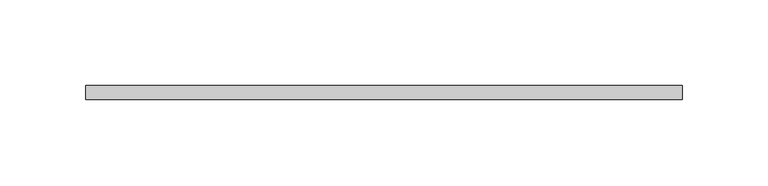
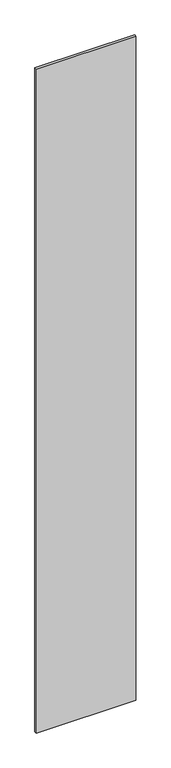
"""IFC4 building model written with IfcOpenShell, lengths in millimetres: proxy geometry, Panel:Panel:300402:Panel:300402 : Panel:Panel:300402:300124:Panel:300402:Panel:300402 : Panel:Panel:300402:300124 : Panel:Panel:300402:Panel:300402 : Panel:Panel:300402:300124:13 : Panel:Panel:300402:Panel:300402 : Panel:Panel:300402:300124:Panel:300402:Panel:300402 : Panel:Panel:300402:300124 : Panel:Panel:300402:Panel:300402 : Panel:Panel:300402:300124:300083."""

from ifc_helpers import new_model, si_unit, frame, origin, place, context, project, spatial, polyline, outline, extrude, source, transform, mapped, element, save


def generic_models_52127762(model_context):
    return source(origin(), model_context, "Body", "SweptSolid", [
        extrude(outline(polyline([(560642.3454126, -579076.8913841), (560642.3454126, -579084.8288841), (560295.8117239, -579084.8288841), (560295.8117239, -579076.8913841), (560642.3454126, -579076.8913841)])), frame((0.0, 0.0, 3695.7), z_axis=(0.0, 0.0, 1.0), x_axis=(1.0, 0.0, 0.0)), (0.0, 0.0, 1.0), 2438.4),
    ])


if __name__ == "__main__":
    model = new_model("IFC4")
    model_context = context("Model", 3, world=origin())
    ifc_project = project(units=[si_unit("LENGTHUNIT", "METRE", prefix="MILLI")], contexts=[model_context])
    site = spatial("IfcSite", under=ifc_project)
    building = spatial("IfcBuilding", under=site)
    placement = place(None, origin())
    generic_models_shape = generic_models_52127762(model_context)
    element("IfcBuildingElementProxy", 1, Name="Panel:Panel:300402:Panel:300402 : Panel:Panel:300402:300124:Panel:300402:Panel:300402 : Panel:Panel:300402:300124 : Panel:Panel:300402:Panel:300402 : Panel:Panel:300402:300124:13 : Panel:Panel:300402:Panel:300402 : Panel:Panel:300402:300124:Panel:300402:Panel:300402 : Panel:Panel:300402:300124 : Panel:Panel:300402:Panel:300402 : Panel:Panel:300402:300124:300083", ObjectType="Panel:Panel:300402:Panel:300402 : Panel:Panel:300402:300124:Panel:300402:Panel:300402 : Panel:Panel:300402:300124 : Panel:Panel:300402:Panel:300402 : Panel:Panel:300402:300124:13 : Panel:Panel:300402:Panel:300402 : Panel:Panel:300402:300124:Panel:300402:Panel:300402 : Panel:Panel:300402:300124 : Panel:Panel:300402:Panel:300402 : Panel:Panel:300402:300124:300083", at=placement, inside=building, context=model_context, shape_type="MappedRepresentation", body=[
        mapped(generic_models_shape, transform((0.0, 0.0, 0.0), x_axis=(1.0, 0.0, 0.0), y_axis=(0.0, 1.0, 0.0), z_axis=(0.0, 0.0, 1.0))),
    ])
    save(model, "model.ifc")

# Revit data of these elements
# Type "Panel:Panel:300402:Panel:300402 : Panel:Panel:300402:300124:Panel:300402:Panel:300402 : Panel:Panel:300402:300124 : Panel:Panel:300402:Panel:300402 : Panel:Panel:300402:300124:13 : Panel:Panel:300402:Panel:300402 : Panel:Panel:300402:300124:Panel:300402:Panel:300402 : Panel:Panel:300402:300124 : Panel:Panel:300402:Panel:300402 : Panel:Panel:300402:300124:300083"
#   NameOverride = "Panel:Panel:300402:Panel:300402 : Panel:Panel:300402:300124:Panel:300402:Panel:300402 : Panel:Panel:300402:300124 : Panel:Panel:300402:Panel:300402 : Panel:Panel:300402:300124:300083"
#   ObjectTypeOverride = "Panel:300402:Panel:300402 : Panel:Panel:300402:300124 : Panel:Panel:300402:Panel:300402 : Panel:Panel:300402:300124"
#   Reference = "Panel"
#   Tag = "300083"
# Element 1 (IfcBuildingElementProxy, "Panel:Panel:300402:Panel:300402 : Panel:Panel:300402:300124:Panel:300402:Panel:300402 : Panel:Panel:300402:300124 : Panel:Panel:300402:Panel:300402 : Panel:Panel:300402:300124:13 : Panel:Panel:300402:Panel:300402 : Panel:Panel:300402:300124:Panel:300402:Panel:300402 : Panel:Panel:300402:300124 : Panel:Panel:300402:Panel:300402 : Panel:Panel:300402:300124:300083")
#   Materials on its faces: "5/16\" PHENOLIC RESIN PANELS (CLASS A FLAME SPREAD) - EXPOSED FASTENERS"
# Materials
#   "5/16\" PHENOLIC RESIN PANELS (CLASS A FLAME SPREAD) - EXPOSED FASTENERS": class "Unassigned", colour RGB 64 64 64, transparency 0, Keynote = "M07420000.01", Cost = 0
